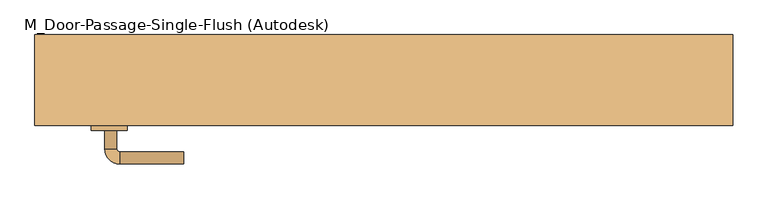
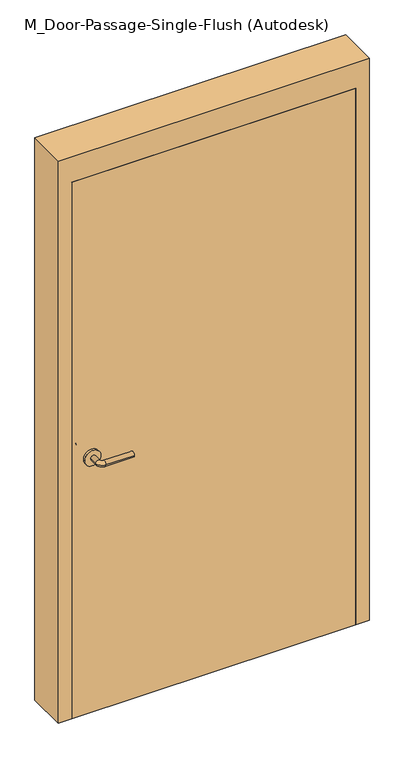
"""IFC4 building model written with IfcOpenShell, lengths in millimetres: door geometry, M_Door-Passage-Single-Flush (Autodesk) : H_DR_AMD_Single Door_Ext_Steel_1050x2100."""

from ifc_helpers import new_model, si_unit, point, frame, frame_2d, origin, origin_with_axes, place, context, project, spatial, polyline, circle_curve, ellipse_curve, trimmed, segment, composite_curve, outline, extrude, faceted_brep, source, transform, mapped, element, save
from ifc_brep_helpers import plane_surface, cylinder_surface, revolved_surface, advanced_brep


def m_door_passage_single_flush_autodesk_9dad06cd(model_context):
    return source(origin(), model_context, "Body", "SolidModel", [
        advanced_brep(
        [(-459.990625, -123.35, 1000.0), (-439.990625, -123.35, 1000.0), (-459.990625, -93.35, 1000.0), (-439.990625, -93.35, 1000.0), (-434.990625, -88.35, 1000.0), (-434.990625, -68.35, 1000.0), (-329.990625, -68.35, 1000.0), (-329.990625, -88.35, 1000.0)],
        [
            (0, 1, circle_curve(frame((-449.990625, -123.35, 1000.0), z_axis=(0.0, -1.0, 0.0), x_axis=(1.0, 0.0, 0.0)), 10.0)),
            (1, 0, circle_curve(frame((-449.990625, -123.35, 1000.0), z_axis=(0.0, -1.0, 0.0), x_axis=(1.0, 0.0, 0.0)), 10.0)),
            (0, 2),
            (2, 3, circle_curve(frame((-449.990625, -93.35, 1000.0), z_axis=(0.0, -1.0, 0.0), x_axis=(1.0, 0.0, 0.0)), 10.0)),
            (3, 1),
            (3, 2, circle_curve(frame((-449.990625, -93.35, 1000.0), z_axis=(0.0, -1.0, 0.0), x_axis=(1.0, 0.0, 0.0)), 10.0)),
            (4, 3, circle_curve(frame((-434.990625, -93.35, 1000.0), z_axis=(0.0, 0.0, 1.0), x_axis=(-1.0, 0.0, 0.0)), 5.0)),
            (2, 5, circle_curve(frame((-434.990625, -93.35, 1000.0), z_axis=(0.0, 0.0, -1.0), x_axis=(-1.0, 0.0, 0.0)), 25.0)),
            (5, 4, circle_curve(frame((-434.990625, -78.35, 1000.0), z_axis=(-1.0, 0.0, 0.0), x_axis=(0.0, -1.0, 0.0)), 10.0)),
            (4, 5, circle_curve(frame((-434.990625, -78.35, 1000.0), z_axis=(-1.0, 0.0, 0.0), x_axis=(0.0, -1.0, 0.0)), 10.0)),
            (6, 7, circle_curve(frame((-329.990625, -78.35, 1000.0), z_axis=(1.0, 0.0, 0.0), x_axis=(0.0, -1.0, 0.0)), 10.0)),
            (7, 6, circle_curve(frame((-329.990625, -78.35, 1000.0), z_axis=(1.0, 0.0, 0.0), x_axis=(0.0, -1.0, 0.0)), 10.0)),
            (5, 6),
            (7, 4),
        ],
        [
            plane_surface(frame((-449.990625, -123.35, 1000.0), z_axis=(0.0, -1.0, 0.0), x_axis=(0.0, 0.0, 1.0))),
            cylinder_surface(frame((-449.990625, -123.35, 1000.0), z_axis=(0.0, -1.0, 0.0), x_axis=(1.0, 0.0, 0.0)), 10.0),
            revolved_surface(trimmed(ellipse_curve(frame((-449.990625, -93.35, 1000.0), z_axis=(0.0, -1.0, 0.0), x_axis=(1.0, 0.0, 0.0)), 10.0, 10.0), [point((-459.990625, -93.35, 1000.0))], [point((-439.990625, -93.35, 1000.0))], True, "CARTESIAN"), (-434.990625, -93.35, 1000.0), (0.0, 0.0, -1.0)),
            revolved_surface(trimmed(ellipse_curve(frame((-449.990625, -93.35, 1000.0), z_axis=(0.0, -1.0, 0.0), x_axis=(1.0, 0.0, 0.0)), 10.0, 10.0), [point((-439.990625, -93.35, 1000.0))], [point((-459.990625, -93.35, 1000.0))], True, "CARTESIAN"), (-434.990625, -93.35, 1000.0), (0.0, 0.0, -1.0)),
            plane_surface(frame((-329.990625, -78.35, 1000.0), z_axis=(1.0, 0.0, 0.0), x_axis=(0.0, 0.0, 1.0))),
            cylinder_surface(frame((-434.990625, -78.35, 1000.0), z_axis=(-1.0, 0.0, 0.0), x_axis=(0.0, -1.0, 0.0)), 10.0),
        ],
        [
            (0, [[1, 2]]),
            (1, [[-1, 3, 4, 5]]),
            (1, [[-2, -5, 6, -3]]),
            (2, [[7, -4, 8, 9]]),
            (3, [[-8, -6, -7, 10]]),
            (4, [[11, 12]]),
            (5, [[-9, 13, -12, 14]]),
            (5, [[-10, -14, -11, -13]]),
        ],
    ),
        extrude(outline(composite_curve([segment(trimmed(circle_curve(frame_2d((1000.0, -452.490625)), 30.0), [point((1000.0, -482.490625))], [point((1000.0, -422.490625))], False, "CARTESIAN"), True, "CONTINUOUS"), segment(trimmed(circle_curve(frame_2d((1000.0, -452.490625)), 30.0), [point((1000.0, -422.490625))], [point((1000.0, -482.490625))], False, "CARTESIAN"), True, "CONTINUOUS")], self_intersect=False)), frame((0.0, -131.35, 0.0), z_axis=(0.0, 1.0, 0.0), x_axis=(0.0, 0.0, 1.0)), (0.0, 0.0, 1.0), 8.0),
        advanced_brep(
        [(-459.990625, -184.35, 1000.0), (-439.990625, -184.35, 1000.0), (-439.990625, -214.35, 1000.0), (-459.990625, -214.35, 1000.0), (-434.990625, -219.35, 1000.0), (-434.990625, -239.35, 1000.0), (-329.990625, -239.35, 1000.0), (-329.990625, -219.35, 1000.0)],
        [
            (0, 1, circle_curve(frame((-449.990625, -184.35, 1000.0), z_axis=(0.0, 1.0, 0.0), x_axis=(1.0, 0.0, 0.0)), 10.0)),
            (1, 0, circle_curve(frame((-449.990625, -184.35, 1000.0), z_axis=(0.0, 1.0, 0.0), x_axis=(1.0, 0.0, 0.0)), 10.0)),
            (1, 2),
            (2, 3, circle_curve(frame((-449.990625, -214.35, 1000.0), z_axis=(0.0, 1.0, 0.0), x_axis=(1.0, 0.0, 0.0)), 10.0)),
            (3, 0),
            (3, 2, circle_curve(frame((-449.990625, -214.35, 1000.0), z_axis=(0.0, 1.0, 0.0), x_axis=(1.0, 0.0, 0.0)), 10.0)),
            (4, 5, circle_curve(frame((-434.990625, -229.35, 1000.0), z_axis=(-1.0, 0.0, 0.0), x_axis=(0.0, 1.0, 0.0)), 10.0)),
            (5, 3, circle_curve(frame((-434.990625, -214.35, 1000.0), z_axis=(0.0, 0.0, -1.0), x_axis=(-1.0, 0.0, 0.0)), 25.0)),
            (2, 4, circle_curve(frame((-434.990625, -214.35, 1000.0), z_axis=(0.0, 0.0, 1.0), x_axis=(-1.0, 0.0, 0.0)), 5.0)),
            (5, 4, circle_curve(frame((-434.990625, -229.35, 1000.0), z_axis=(-1.0, 0.0, 0.0), x_axis=(0.0, 1.0, 0.0)), 10.0)),
            (6, 7, circle_curve(frame((-329.990625, -229.35, 1000.0), z_axis=(1.0, 0.0, 0.0), x_axis=(0.0, 1.0, 0.0)), 10.0)),
            (7, 6, circle_curve(frame((-329.990625, -229.35, 1000.0), z_axis=(1.0, 0.0, 0.0), x_axis=(0.0, 1.0, 0.0)), 10.0)),
            (4, 7),
            (6, 5),
        ],
        [
            plane_surface(frame((-449.990625, -184.35, 1000.0), z_axis=(0.0, 1.0, 0.0), x_axis=(0.0, 0.0, 1.0))),
            cylinder_surface(frame((-449.990625, -184.35, 1000.0), z_axis=(0.0, 1.0, 0.0), x_axis=(1.0, 0.0, 0.0)), 10.0),
            revolved_surface(trimmed(ellipse_curve(frame((-449.990625, -214.35, 1000.0), z_axis=(0.0, -1.0, 0.0), x_axis=(1.0, 0.0, 0.0)), 10.0, 10.0), [point((-459.990625, -214.35, 1000.0))], [point((-439.990625, -214.35, 1000.0))], True, "CARTESIAN"), (-434.990625, -214.35, 1000.0), (0.0, 0.0, -1.0)),
            revolved_surface(trimmed(ellipse_curve(frame((-449.990625, -214.35, 1000.0), z_axis=(0.0, -1.0, 0.0), x_axis=(1.0, 0.0, 0.0)), 10.0, 10.0), [point((-439.990625, -214.35, 1000.0))], [point((-459.990625, -214.35, 1000.0))], True, "CARTESIAN"), (-434.990625, -214.35, 1000.0), (0.0, 0.0, -1.0)),
            plane_surface(frame((-329.990625, -229.35, 1000.0), z_axis=(1.0, 0.0, 0.0), x_axis=(0.0, 0.0, 1.0))),
            cylinder_surface(frame((-434.990625, -229.35, 1000.0), z_axis=(-1.0, 0.0, 0.0), x_axis=(0.0, 1.0, 0.0)), 10.0),
        ],
        [
            (0, [[1, 2]]),
            (1, [[3, 4, 5, -2]]),
            (1, [[-5, 6, -3, -1]]),
            (2, [[7, 8, -4, 9]]),
            (3, [[10, -9, -6, -8]]),
            (4, [[11, 12]]),
            (5, [[13, -11, 14, -7]]),
            (5, [[-14, -12, -13, -10]]),
        ],
    ),
        extrude(outline(composite_curve([segment(trimmed(circle_curve(frame_2d((1000.0, -452.490625)), 30.0), [point((1000.0, -482.490625))], [point((1000.0, -422.490625))], False, "CARTESIAN"), True, "CONTINUOUS"), segment(trimmed(circle_curve(frame_2d((1000.0, -452.490625)), 30.0), [point((1000.0, -422.490625))], [point((1000.0, -482.490625))], False, "CARTESIAN"), True, "CONTINUOUS")], self_intersect=False)), frame((0.0, -184.35, 0.0), z_axis=(0.0, 1.0, 0.0), x_axis=(0.0, 0.0, 1.0)), (0.0, 0.0, 1.0), 8.0),
        faceted_brep([(525.0, -126.5875, 0.0), (509.125, -126.5875, 0.0), (509.125, -75.5625, 0.0), (525.0, -75.5625, 0.0), (525.0, -26.35, 0.0), (575.0, -26.35, 0.0), (575.0, -176.35, 0.0), (525.0, -176.35, 0.0), (525.0, -176.35, 2100.0), (525.0, -126.5875, 2100.0), (575.0, -176.35, 2200.0), (-575.0, -176.35, 2200.0), (-575.0, -176.35, 0.0), (-525.0, -176.35, 0.0), (-525.0, -176.35, 2100.0), (575.0, -26.35, 2200.0), (525.0, -26.35, 2100.0), (-525.0, -26.35, 2100.0), (-525.0, -26.35, 0.0), (-575.0, -26.35, 0.0), (-575.0, -26.35, 2200.0), (525.0, -75.5625, 2100.0), (509.125, -75.5625, 2084.125), (-509.125, -75.5625, 2084.125), (-509.125, -75.5625, 0.0), (-525.0, -75.5625, 0.0), (-525.0, -75.5625, 2100.0), (509.125, -126.5875, 2084.125), (-525.0, -126.5875, 2100.0), (-525.0, -126.5875, 0.0), (-509.125, -126.5875, 0.0), (-509.125, -126.5875, 2084.125)], [[[0, 1, 2, 3, 4, 5, 6, 7]], [[7, 8, 9, 0]], [[6, 10, 11, 12, 13, 14, 8, 7]], [[5, 15, 10, 6]], [[4, 16, 17, 18, 19, 20, 15, 5]], [[3, 21, 16, 4]], [[2, 22, 23, 24, 25, 26, 21, 3]], [[1, 27, 22, 2]], [[0, 9, 28, 29, 30, 31, 27, 1]], [[8, 14, 28, 9]], [[16, 21, 26, 17]], [[22, 27, 31, 23]], [[12, 19, 18, 25, 24, 30, 29, 13]], [[13, 29, 28, 14]], [[11, 20, 19, 12]], [[17, 26, 25, 18]], [[23, 31, 30, 24]], [[15, 20, 11, 10]]]),
        extrude(outline(polyline([(525.0, -131.35), (525.0, -176.35), (-525.0, -176.35), (-525.0, -131.35), (525.0, -131.35)])), origin_with_axes(), (0.0, 0.0, 1.0), 2100.0),
    ])


if __name__ == "__main__":
    model = new_model("IFC4")
    model_context = context("Model", 3, world=origin())
    ifc_project = project(units=[si_unit("LENGTHUNIT", "METRE", prefix="MILLI")], contexts=[model_context])
    site = spatial("IfcSite", under=ifc_project)
    building = spatial("IfcBuilding", under=site)
    placement = place(None, origin())
    m_door_passage_single_flush_autodesk_shape = m_door_passage_single_flush_autodesk_9dad06cd(model_context)
    element("IfcDoor", 1, ObjectType="M_Door-Passage-Single-Flush (Autodesk) : H_DR_AMD_Single Door_Ext_Steel_1050x2100", at=placement, inside=building, context=model_context, shape_type="MappedRepresentation", body=[
        mapped(m_door_passage_single_flush_autodesk_shape, transform((0.0, 0.0, 0.0), x_axis=(1.0, 0.0, 0.0), y_axis=(0.0, 1.0, 0.0), z_axis=(0.0, 0.0, 1.0))),
    ])
    save(model, "model.ifc")

# Revit data of these elements
# Type "M_Door-Passage-Single-Flush (Autodesk) : H_DR_AMD_Single Door_Ext_Steel_1050x2100"
#   Type Mark = "SD"
#   Assembly Code = "B2030200"
#   Analytic Construction = "Wooden"
#   Thickness = 0.0450 m
#   Thermal Resistance (R) = 0.455703 (m²·K)/W
#   Swing Angle [instance default] = 90.00°
#   Strike Height = 1.0000 m
#   Rough Width [instance default] = 1.1500 m
#   Rough Height [instance default] = 2.2000 m
#   MF Opening Height [instance default] = 0.1000 m
#   MF Opening Width [instance default] = 0.1000 m
#   Inset Calculate [instance default] = 0.1050 m
#   Masonry Inset [instance default] = 0.0250 m
#   Height = 2.1000 m
#   Width = 1.0500 m
#   Heat Transfer Coefficient (U) = 2.19465 W/(m²·K)
#   Masonry Frame Depth = 0.1500 m
#   Masonry Frame [instance default] = yes
#   Function = 1
#   Dry Wall Frame [instance default] = no
#   Panel Material = Metal - Steel
#   Frame Material = Metal - Paint Finish - Grey
#   Door Handle Material = Aluminum
#   Visual Light Transmittance = 0
#   Solar Heat Gain Coefficient = 0
#   Wall Closure = (empty or 0)
# Element 1 (IfcDoor, "M_Door-Passage-Single-Flush (Autodesk) : H_DR_AMD_Single Door_Ext_Steel_1050x2100")
#   Materials on its faces: "Aluminum", "Metal - Paint Finish - Grey", "Metal - Steel"
# Materials
#   "Metal - Steel": class "Metal", colour RGB 247 247 247, transparency 0, Cost = 0
#   "Metal - Paint Finish - Grey": class "Paint", colour RGB 104 104 104, transparency 0, Cost = 0
#   "Aluminum": class "Metal", colour RGB 244 244 244, transparency 0, Description = "Aluminum 6061", Cost = 0
